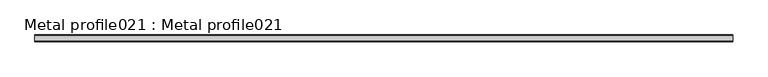
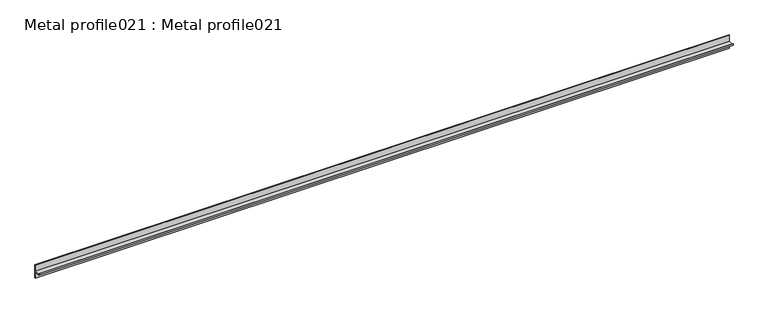
"""IFC4 building model written with IfcOpenShell, lengths in millimetres: proxy geometry, Metal profile021 : Metal profile021."""

from ifc_helpers import new_model, si_unit, frame, origin, place, context, project, spatial, polyline, outline, extrude, source, transform, mapped, element, save


def metal_profile021_metal_profile021_f5a32519(model_context):
    return source(origin(), model_context, "Body", "SweptSolid", [
        extrude(outline(polyline([(-4684.6182816, 39055.86375), (-4667.6543336, 39055.86375), (-4667.6543336, 39074.91375), (-4666.3843336, 39074.91375), (-4666.3843336, 39035.54375), (-4667.6543336, 39035.54375), (-4667.6543336, 39054.59375), (-4685.8882816, 39054.59375), (-4685.8882816, 39059.34355), (-4684.6182816, 39059.34355), (-4684.6182816, 39055.86375)])), frame((12383.0178845, 0.0, 0.0), z_axis=(1.0, 0.0, 0.0), x_axis=(0.0, 1.0, 0.0)), (0.0, 0.0, 1.0), 2000.0),
    ])


if __name__ == "__main__":
    model = new_model("IFC4")
    model_context = context("Model", 3, world=origin())
    ifc_project = project(units=[si_unit("LENGTHUNIT", "METRE", prefix="MILLI")], contexts=[model_context])
    site = spatial("IfcSite", under=ifc_project)
    building = spatial("IfcBuilding", under=site)
    placement = place(None, origin())
    metal_profile021_metal_profile021_shape = metal_profile021_metal_profile021_f5a32519(model_context)
    element("IfcBuildingElementProxy", 1, Name="Metal profile021 : Metal profile021", ObjectType="Metal profile021 : Metal profile021", at=placement, inside=building, context=model_context, shape_type="MappedRepresentation", body=[
        mapped(metal_profile021_metal_profile021_shape, transform((0.0, 0.0, 0.0), x_axis=(1.0, 0.0, 0.0), y_axis=(0.0, 1.0, 0.0), z_axis=(0.0, 0.0, 1.0))),
    ])
    save(model, "model.ifc")

# Revit data of these elements
# Type "Metal profile021 : Metal profile021"
#   NameOverride = "Metal profile021"
# Element 1 (IfcBuildingElementProxy, "Metal profile021 : Metal profile021")
#   Materials on its faces: "16 GA. COPPER VENTED T REVEAL BEAD"
# Materials
#   "16 GA. COPPER VENTED T REVEAL BEAD": class "Unassigned", colour RGB 255 227 10, transparency 0
